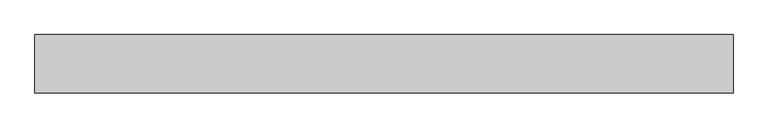
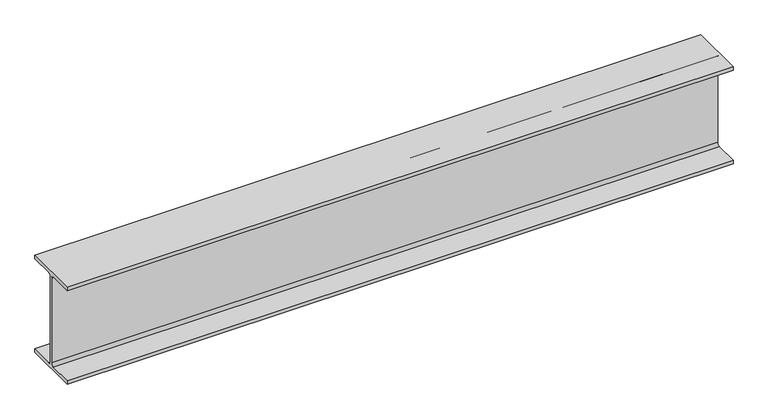
"""IFC4 building model written with IfcOpenShell, lengths in millimetres: beam geometry, Old_Steel Beam_H-KSD3502 : H_SB_ASB_H-194×150x6x9."""

from ifc_helpers import new_model, si_unit, point, frame, frame_2d, origin, place, context, project, spatial, polyline, circle_curve, trimmed, segment, composite_curve, outline, extrude, source, transform, mapped, element, save


def beam_a4e83b10(model_context):
    return source(origin(), model_context, "Body", "SweptSolid", [
        extrude(outline(composite_curve([segment(polyline([(-82.5, -141.5), (-11.9, -141.5)]), True, "CONTINUOUS"), segment(trimmed(circle_curve(frame_2d((-11.9, -132.6)), 8.9), [point((-11.9, -141.5))], [point((-3.0, -132.6))], True, "CARTESIAN"), True, "CONTINUOUS"), segment(polyline([(-3.0, -132.6), (-3.0, 132.6)]), True, "CONTINUOUS"), segment(trimmed(circle_curve(frame_2d((-11.9, 132.6)), 8.9), [point((-3.0, 132.6))], [point((-11.9, 141.5))], True, "CARTESIAN"), True, "CONTINUOUS"), segment(polyline([(-11.9, 141.5), (-82.5, 141.5), (-82.5, 151.7), (82.5, 151.7), (82.5, 141.5), (11.9, 141.5)]), True, "CONTINUOUS"), segment(trimmed(circle_curve(frame_2d((11.9, 132.6)), 8.9), [point((11.9, 141.5))], [point((3.0, 132.6))], True, "CARTESIAN"), True, "CONTINUOUS"), segment(polyline([(3.0, 132.6), (3.0, -132.6)]), True, "CONTINUOUS"), segment(trimmed(circle_curve(frame_2d((11.9, -132.6)), 8.9), [point((3.0, -132.6))], [point((11.9, -141.5))], True, "CARTESIAN"), True, "CONTINUOUS"), segment(polyline([(11.9, -141.5), (82.5, -141.5), (82.5, -151.7), (-82.5, -151.7), (-82.5, -141.5)]), True, "CONTINUOUS")], self_intersect=False)), frame((-988.3546085, 0.0, 0.0), z_axis=(1.0, 0.0, 0.0), x_axis=(0.0, 1.0, 0.0)), (0.0, 0.0, 1.0), 1976.709217),
    ])


if __name__ == "__main__":
    model = new_model("IFC4")
    model_context = context("Model", 3, world=origin())
    ifc_project = project(units=[si_unit("LENGTHUNIT", "METRE", prefix="MILLI")], contexts=[model_context])
    site = spatial("IfcSite", under=ifc_project)
    building = spatial("IfcBuilding", under=site)
    placement = place(None, origin())
    beam_shape = beam_a4e83b10(model_context)
    element("IfcBeam", 1, ObjectType="Old_Steel Beam_H-KSD3502 : H_SB_ASB_H-194×150x6x9", at=placement, inside=building, context=model_context, shape_type="MappedRepresentation", body=[
        mapped(beam_shape, transform((0.0, 0.0, 0.0), x_axis=(1.0, 0.0, 0.0), y_axis=(0.0, 1.0, 0.0), z_axis=(0.0, 0.0, 1.0))),
    ])
    save(model, "model.ifc")

# Revit data of these elements
# Type "Old_Steel Beam_H-KSD3502 : H_SB_ASB_H-194×150x6x9"
#   Width = 15.0 cm
#   Web Thickness = 0.6 cm
#   Web Fillet = 1.3 cm
#   Warping Constant = 43316.0 cm⁶
#   Torsional Moment of Inertia = 8.622 cm⁴
#   Torsional Modulus = 1.0 cm³
#   Section Area = 39.01 cm²
#   Plastic Modulus weak axis = 104.0 cm³
#   Plastic Modulus strong axis = 309.0 cm³
#   Perimeter = 0.95 m²/m
#   Nominal Weight = 30.60 kgf/m
#   Moment of Inertia weak axis = 507.00 cm⁴
#   Moment of Inertia strong axis = 2690.00 cm⁴
#   Height = 19.4 cm
#   Flange Thickness = 0.9 cm
#   Elastic Modulus weak axis = 67.6 cm³
#   Elastic Modulus strong axis = 277.0 cm³
#   Centroid Vertical = 9.7 cm
#   Centroid Horizontal = 7.5 cm
#   Length [instance default] = 1.5240 m
#   Structural Material [instance default] = Steel, 45-345
#   Assembly Code = ""
# Element 1 (IfcBeam, "Old_Steel Beam_H-KSD3502 : H_SB_ASB_H-194×150x6x9")
#   Structural Material = none
# Materials
#   "Steel, 45-345": class "Metal", colour RGB 189 187 185, transparency 0, Description = "Steel 345 MPa", Cost = 0
